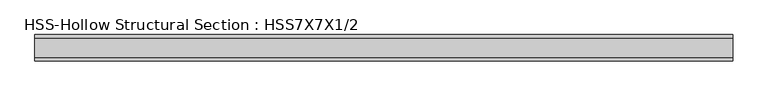
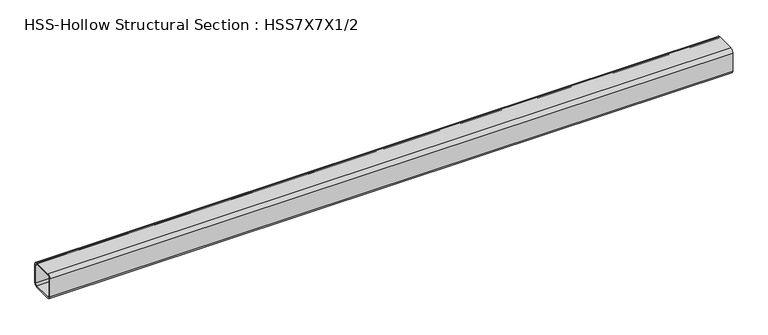
"""IFC4 building model written with IfcOpenShell, lengths in millimetres: member geometry, HSS-Hollow Structural Section : HSS7X7X1/2."""

from ifc_helpers import new_model, si_unit, point, frame, frame_2d, origin, place, context, project, spatial, polyline, circle_curve, trimmed, segment, composite_curve, outline, extrude, source, transform, mapped, element, save


def hss_hollow_structural_section_hss7x7x1_2_92c05659(model_context):
    return source(origin(), model_context, "Body", "SweptSolid", [
        extrude(outline(composite_curve([segment(polyline([(88.9, 65.278), (88.9, -65.278)]), True, "CONTINUOUS"), segment(trimmed(circle_curve(frame_2d((65.278, -65.278)), 23.622), [point((88.9, -65.278))], [point((65.278, -88.9))], False, "CARTESIAN"), True, "CONTINUOUS"), segment(polyline([(65.278, -88.9), (-65.278, -88.9)]), True, "CONTINUOUS"), segment(trimmed(circle_curve(frame_2d((-65.278, -65.278)), 23.622), [point((-65.278, -88.9))], [point((-88.9, -65.278))], False, "CARTESIAN"), True, "CONTINUOUS"), segment(polyline([(-88.9, -65.278), (-88.9, 65.278)]), True, "CONTINUOUS"), segment(trimmed(circle_curve(frame_2d((-65.278, 65.278)), 23.622), [point((-88.9, 65.278))], [point((-65.278, 88.9))], False, "CARTESIAN"), True, "CONTINUOUS"), segment(polyline([(-65.278, 88.9), (65.278, 88.9)]), True, "CONTINUOUS"), segment(trimmed(circle_curve(frame_2d((65.278, 65.278)), 23.622), [point((65.278, 88.9))], [point((88.9, 65.278))], False, "CARTESIAN"), True, "CONTINUOUS")], self_intersect=False), holes=[composite_curve([segment(trimmed(circle_curve(frame_2d((-65.278, 65.278)), 11.811), [point((-65.278, 77.089))], [point((-77.089, 65.278))], True, "CARTESIAN"), True, "CONTINUOUS"), segment(polyline([(-77.089, 65.278), (-77.089, -65.278)]), True, "CONTINUOUS"), segment(trimmed(circle_curve(frame_2d((-65.278, -65.278)), 11.811), [point((-77.089, -65.278))], [point((-65.278, -77.089))], True, "CARTESIAN"), True, "CONTINUOUS"), segment(polyline([(-65.278, -77.089), (65.278, -77.089)]), True, "CONTINUOUS"), segment(trimmed(circle_curve(frame_2d((65.278, -65.278)), 11.811), [point((65.278, -77.089))], [point((77.089, -65.278))], True, "CARTESIAN"), True, "CONTINUOUS"), segment(polyline([(77.089, -65.278), (77.089, 65.278)]), True, "CONTINUOUS"), segment(trimmed(circle_curve(frame_2d((65.278, 65.278)), 11.811), [point((77.089, 65.278))], [point((65.278, 77.089))], True, "CARTESIAN"), True, "CONTINUOUS"), segment(polyline([(65.278, 77.089), (-65.278, 77.089)]), True, "CONTINUOUS")], self_intersect=False)]), frame((-2119.0722905, 0.0, 0.0), z_axis=(1.0, 0.0, 0.0), x_axis=(0.0, 1.0, 0.0)), (0.0, 0.0, 1.0), 4689.9710714),
    ])


if __name__ == "__main__":
    model = new_model("IFC4")
    model_context = context("Model", 3, world=origin())
    ifc_project = project(units=[si_unit("LENGTHUNIT", "METRE", prefix="MILLI")], contexts=[model_context])
    site = spatial("IfcSite", under=ifc_project)
    building = spatial("IfcBuilding", under=site)
    placement = place(None, origin())
    hss_hollow_structural_section_hss7x7x1_2_shape = hss_hollow_structural_section_hss7x7x1_2_92c05659(model_context)
    element("IfcMember", 1, ObjectType="HSS-Hollow Structural Section : HSS7X7X1/2", at=placement, inside=building, context=model_context, shape_type="MappedRepresentation", body=[
        mapped(hss_hollow_structural_section_hss7x7x1_2_shape, transform((0.0, 0.0, 0.0), x_axis=(1.0, 0.0, 0.0), y_axis=(0.0, 1.0, 0.0), z_axis=(0.0, 0.0, 1.0))),
    ])
    save(model, "model.ifc")

# Revit data of these elements
# Type "HSS-Hollow Structural Section : HSS7X7X1/2"
#   Assembly Code = "B10"
#   Shape = "Square"
#   W = 41.9
#   Ht = 0' - 7"
#   Length [instance default] = 5' - 0"
#   b = 0' - 7"
#   kr = 0' - 0.93"
#   t = 0' - 0.465"
#   A = 0.0805556 SF
#   Structural Material [instance default] = Steel ASTM A500, Grade B, Rectangular and Square
# Element 1 (IfcMember, "HSS-Hollow Structural Section : HSS7X7X1/2")
#   Materials on its faces: "Steel ASTM A500, Grade B, Rectangular and Square"
# Materials
#   "Steel ASTM A500, Grade B, Rectangular and Square": class "Metal", colour RGB 199 199 199, transparency 0, Description = "Carbon steel", Cost = 0
